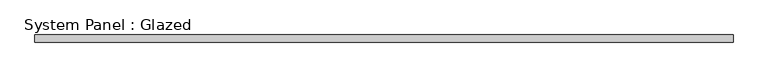
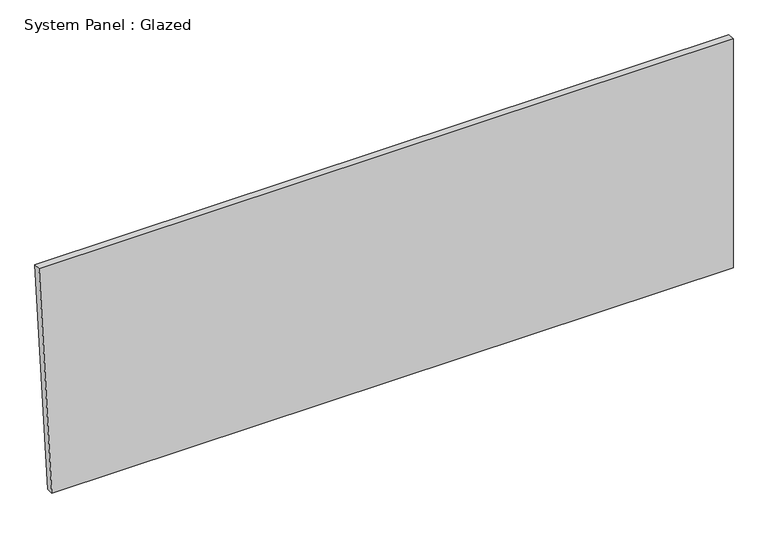
"""IFC4 building model written with IfcOpenShell, lengths in millimetres: plate geometry, System Panel : Glazed."""

from ifc_helpers import new_model, si_unit, frame, origin, place, context, project, spatial, polyline, outline, extrude, source, transform, mapped, element, save


def system_panel_glazed_f82295e9(model_context):
    return source(origin(), model_context, "Body", "SweptSolid", [
        extrude(outline(polyline([(0.0, -1197.3859051), (0.0, 1242.7131117), (866.081558, 1242.7131117), (866.081558, -1242.7131117), (0.0, -1197.3859051)])), frame((0.0, -44.45, 0.0), z_axis=(0.0, 1.0, 0.0), x_axis=(0.0, 0.0, 1.0)), (0.0, 0.0, 1.0), 25.4),
    ])


if __name__ == "__main__":
    model = new_model("IFC4")
    model_context = context("Model", 3, world=origin())
    ifc_project = project(units=[si_unit("LENGTHUNIT", "METRE", prefix="MILLI")], contexts=[model_context])
    site = spatial("IfcSite", under=ifc_project)
    building = spatial("IfcBuilding", under=site)
    placement = place(None, origin())
    system_panel_glazed_shape = system_panel_glazed_f82295e9(model_context)
    element("IfcPlate", 1, ObjectType="System Panel : Glazed", at=placement, inside=building, context=model_context, shape_type="MappedRepresentation", body=[
        mapped(system_panel_glazed_shape, transform((0.0, 0.0, 0.0), x_axis=(1.0, 0.0, 0.0), y_axis=(0.0, 1.0, 0.0), z_axis=(0.0, 0.0, 1.0))),
    ])
    save(model, "model.ifc")

# Revit data of these elements
# Type "System Panel : Glazed"
#   Construction Type Id = "GSP4R"
#   Analytic Construction = "1/8 in Pilkington single glazing"
#   Visual Light Transmittance = 0.9
#   Solar Heat Gain Coefficient = 0.86
#   Heat Transfer Coefficient (U) = 1.18115 BTU/(h·ft²·°F)
#   Define Thermal Properties by = 1
# Element 1 (IfcPlate, "System Panel : Glazed")
#   Materials on its faces: "Glass"
# Materials
#   "Glass": class "Glass", colour RGB 0 128 192, transparency 0.75, Description = "Soda Lime Glass", Cost = 0
